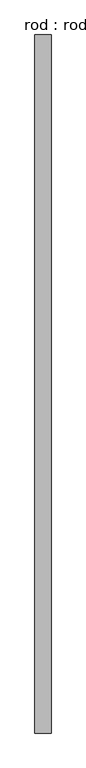
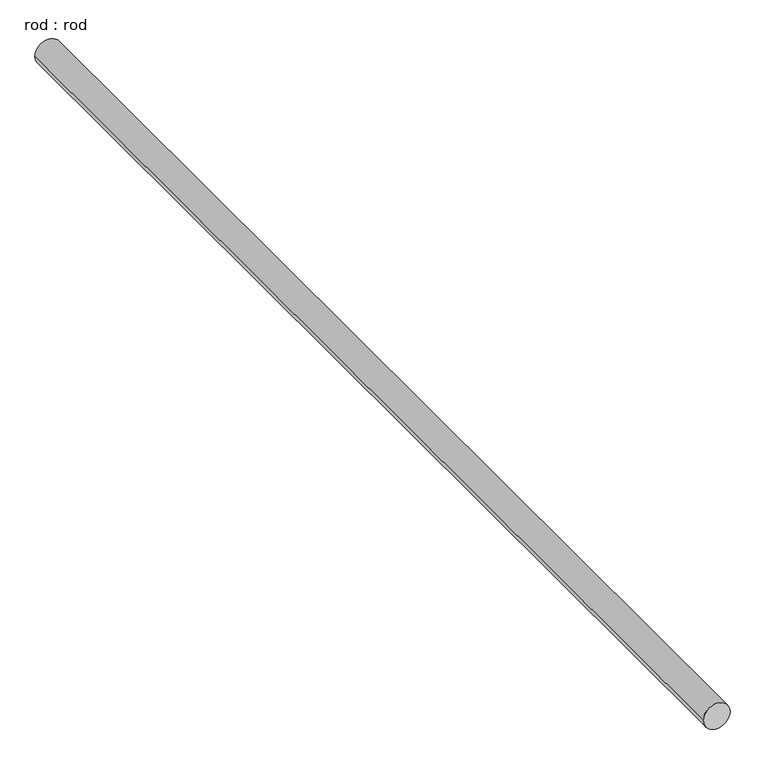
"""IFC4 building model written with IfcOpenShell, lengths in millimetres: proxy geometry, rod : rod."""

from ifc_helpers import new_model, si_unit, point, frame, frame_2d, origin, place, context, project, spatial, circle_curve, trimmed, segment, composite_curve, outline, extrude, source, transform, mapped, element, save


def rod_rod_b6f56cd7(model_context):
    return source(origin(), model_context, "Body", "SweptSolid", [
        extrude(outline(composite_curve([segment(trimmed(circle_curve(frame_2d((0.0108462, 0.0)), 200.0), [point((0.0108462, 200.0))], [point((0.0108462, -200.0))], False, "CARTESIAN"), True, "CONTINUOUS"), segment(trimmed(circle_curve(frame_2d((0.0108462, 0.0)), 200.0), [point((0.0108462, -200.0))], [point((0.0108462, 200.0))], False, "CARTESIAN"), True, "CONTINUOUS")], self_intersect=False)), frame((0.0, -4558.2381056, 0.0), z_axis=(0.0, 1.0, 0.0), x_axis=(0.0, 0.0, 1.0)), (0.0, 0.0, 1.0), 17301.9334419),
    ])


if __name__ == "__main__":
    model = new_model("IFC4")
    model_context = context("Model", 3, world=origin())
    ifc_project = project(units=[si_unit("LENGTHUNIT", "METRE", prefix="MILLI")], contexts=[model_context])
    site = spatial("IfcSite", under=ifc_project)
    building = spatial("IfcBuilding", under=site)
    placement = place(None, origin())
    rod_rod_shape = rod_rod_b6f56cd7(model_context)
    element("IfcBuildingElementProxy", 1, Name="rod : rod", ObjectType="rod : rod", at=placement, inside=building, context=model_context, shape_type="MappedRepresentation", body=[
        mapped(rod_rod_shape, transform((0.0, 0.0, 0.0), x_axis=(1.0, 0.0, 0.0), y_axis=(0.0, 1.0, 0.0), z_axis=(0.0, 0.0, 1.0))),
    ])
    save(model, "model.ifc")

# Revit data of these elements
# Type "rod : rod"
#   Default Elevation = 0
